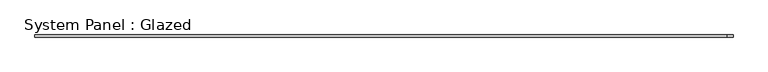
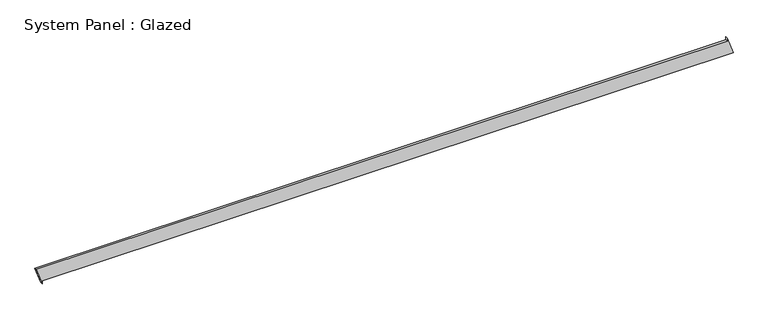
"""IFC4 building model written with IfcOpenShell, lengths in millimetres: plate geometry, System Panel : Glazed."""

import ifcopenshell
import ifcopenshell.guid

model = None  # the IFC model being written
_history = None  # IfcOwnerHistory: only IFC2X3 demands one
_inside = {}  # id of a spatial element -> (the spatial element, [elements in it])
_under = {}  # id of a project, library or spatial element -> (it, [spatial elements below it])
_declared = {}  # id of a project -> (the project, [libraries it declares])
_typed = {}  # id of a type object -> (the type object, [elements of that type])
_made_of = {}  # id of a material, layer set ... -> (it, [elements and type objects made of it])


def new_model(schema):
    """Start an empty IFC model of exactly this schema.

    Asked for "IFC4X3", IfcOpenShell would pick the latest addendum, in which some entities
    have other attributes; the version numbers below select the first issue.
    IFC2X3 requires an IfcOwnerHistory on every rooted entity: one is made here for all.
    """
    global model, _history
    if schema == "IFC4X3":
        model = ifcopenshell.file(schema_version=(4, 3, 0, 0))
    else:
        model = ifcopenshell.file(schema=schema)
    _inside.clear()
    _under.clear()
    _declared.clear()
    _typed.clear()
    _made_of.clear()
    _history = None
    if model.schema == "IFC2X3":
        org = make("IfcOrganization", Name="unknown")
        user = make(
            "IfcPersonAndOrganization",
            ThePerson=make("IfcPerson", FamilyName="unknown"),
            TheOrganization=org,
        )
        app = make(
            "IfcApplication",
            ApplicationDeveloper=org,
            Version="unknown",
            ApplicationFullName="unknown",
            ApplicationIdentifier="unknown",
        )
        _history = make(
            "IfcOwnerHistory",
            OwningUser=user,
            OwningApplication=app,
            ChangeAction="ADDED",
            CreationDate=0,
        )
    return model


def make(cls, **values):
    """One entity of the class cls with the attributes given. An attribute that is None is left unset."""
    return model.create_entity(
        cls, **{name: value for name, value in values.items() if value is not None}
    )


def rooted(cls, **values):
    """An entity with a GlobalId (a new one), such as an element, a storey or a relation."""
    return make(cls, GlobalId=ifcopenshell.guid.new(), OwnerHistory=_history, **values)


def si_unit(unit_type, name, prefix=None):
    """IfcSIUnit, for example si_unit("LENGTHUNIT", "METRE", prefix="MILLI")."""
    return make("IfcSIUnit", UnitType=unit_type, Prefix=prefix, Name=name)


def assignment(units):
    """IfcUnitAssignment: the units of a project."""
    return None if units is None else make("IfcUnitAssignment", Units=units)


def point(xyz):
    """IfcCartesianPoint."""
    return None if xyz is None else make("IfcCartesianPoint", Coordinates=xyz)


def direction(xyz):
    """IfcDirection."""
    return None if xyz is None else make("IfcDirection", DirectionRatios=xyz)


def frame(location, z_axis=None, x_axis=None):
    """IfcAxis2Placement3D, a coordinate frame: its origin and axes. An axis left out is left unset."""
    return make(
        "IfcAxis2Placement3D",
        Location=point(location),
        Axis=direction(z_axis),
        RefDirection=direction(x_axis),
    )


def origin():
    """The frame at (0, 0, 0) with its axes left unset."""
    return frame((0.0, 0.0, 0.0))


def place(relative_to, where):
    """IfcLocalPlacement: puts the frame where relative to a parent placement (None: the world)."""
    return make(
        "IfcLocalPlacement", PlacementRelTo=relative_to, RelativePlacement=where
    )


def context(
    kind, dimensions, precision=None, world=None, true_north=None, identifier=None
):
    """IfcGeometricRepresentationContext, for example the 3D "Model" context."""
    return make(
        "IfcGeometricRepresentationContext",
        ContextIdentifier=identifier,
        ContextType=kind,
        CoordinateSpaceDimension=dimensions,
        Precision=precision,
        WorldCoordinateSystem=world,
        TrueNorth=true_north,
    )


def project(units=None, contexts=None):
    """IfcProject with its units and contexts."""
    return rooted(
        "IfcProject",
        Name="project",
        RepresentationContexts=contexts,
        UnitsInContext=assignment(units),
    )


def spatial(cls, under=None, at=None, **own):
    """A site, building, storey or space (cls), placed at a placement, below another one or the project."""
    s = rooted(cls, ObjectPlacement=at, **own)
    if under is not None:
        _under.setdefault(under.id(), (under, []))[1].append(s)
    return s


def polyline(points):
    """IfcPolyline through the points."""
    return make("IfcPolyline", Points=[point(p) for p in points])


def outline(outer, holes=None, kind="AREA"):
    """IfcArbitraryClosedProfileDef: a profile drawn as a closed curve; with holes, ...WithVoids."""
    if holes is None:
        return make("IfcArbitraryClosedProfileDef", ProfileType=kind, OuterCurve=outer)
    return make(
        "IfcArbitraryProfileDefWithVoids",
        ProfileType=kind,
        OuterCurve=outer,
        InnerCurves=holes,
    )


def extrude(swept, where, along, depth):
    """IfcExtrudedAreaSolid: the profile swept, set in the frame where, extruded along a direction by depth."""
    return make(
        "IfcExtrudedAreaSolid",
        SweptArea=swept,
        Position=where,
        ExtrudedDirection=direction(along),
        Depth=depth,
    )


def shape(context_of_items, identifier, shape_type, items):
    """IfcShapeRepresentation: the items that make up one representation, for example the "Body"."""
    return make(
        "IfcShapeRepresentation",
        ContextOfItems=context_of_items,
        RepresentationIdentifier=identifier,
        RepresentationType=shape_type,
        Items=items,
    )


def source(mapping_origin, context_of_items, identifier, shape_type, items):
    """IfcRepresentationMap: a shape defined once, which mapped items show again and again."""
    return make(
        "IfcRepresentationMap",
        MappingOrigin=mapping_origin,
        MappedRepresentation=shape(context_of_items, identifier, shape_type, items),
    )


def transform(
    local_origin,
    x_axis=None,
    y_axis=None,
    z_axis=None,
    scale=None,
    scale2=None,
    scale3=None,
    uniform=True,
):
    """IfcCartesianTransformationOperator3D, or its non-uniform kind. x_axis, y_axis, z_axis: its Axis1, 2, 3."""
    if uniform:
        return make(
            "IfcCartesianTransformationOperator3D",
            Axis1=direction(x_axis),
            Axis2=direction(y_axis),
            LocalOrigin=point(local_origin),
            Scale=scale,
            Axis3=direction(z_axis),
        )
    return make(
        "IfcCartesianTransformationOperator3DnonUniform",
        Axis1=direction(x_axis),
        Axis2=direction(y_axis),
        LocalOrigin=point(local_origin),
        Scale=scale,
        Axis3=direction(z_axis),
        Scale2=scale2,
        Scale3=scale3,
    )


def mapped(mapping_source, mapping_target):
    """IfcMappedItem: shows the shape of a source again, moved by a transform."""
    return make(
        "IfcMappedItem", MappingSource=mapping_source, MappingTarget=mapping_target
    )


def made_of(thing, what):
    """Note that an element or type object is made of a material, layer set ...; save() writes the relation."""
    if what is not None:
        _made_of.setdefault(what.id(), (what, []))[1].append(thing)
    return thing


def element(
    cls,
    number,
    at=None,
    inside=None,
    cuts=None,
    type_object=None,
    material=None,
    context=None,
    identifier="Body",
    shape_type=None,
    held_by="IfcProductDefinitionShape",
    body=None,
    shapes=None,
    **own,
):
    """One element of the class cls, such as IfcWall. Its Tag is "e" and its number.

    at: its placement. inside: the storey or other place that contains it. cuts: it is an
    opening in that element (IfcRelVoidsElement). A single representation is given by context,
    identifier, shape_type and body (its items); several are given by shapes. held_by: the class
    of the entity that holds the representations. save() writes the other relations.
    """
    e = rooted(cls, Tag="e%d" % number, ObjectPlacement=at, **own)
    if body is not None:
        shapes = [shape(context, identifier, shape_type, body)]
    if shapes is not None:
        e.Representation = make(held_by, Representations=shapes)
    if inside is not None:
        _inside.setdefault(inside.id(), (inside, []))[1].append(e)
    if cuts is not None:
        rooted(
            "IfcRelVoidsElement", RelatingBuildingElement=cuts, RelatedOpeningElement=e
        )
    if type_object is not None:
        _typed.setdefault(type_object.id(), (type_object, []))[1].append(e)
    return made_of(e, material)


def aggregate(whole, parts):
    """IfcRelAggregates: a whole, such as a stair, and the parts it consists of."""
    return rooted("IfcRelAggregates", RelatingObject=whole, RelatedObjects=parts)


def save(model, path):
    """Write the relations noted so far, then the file.

    IfcRelAggregates (storeys below a building ...), IfcRelContainedInSpatialStructure (elements
    in a storey), IfcRelDefinesByType, IfcRelAssociatesMaterial and IfcRelDeclares: one each for
    every whole, place, type object, material and project.
    """
    for whole, parts in _under.values():
        aggregate(whole, parts)
    for where, things in _inside.values():
        rooted(
            "IfcRelContainedInSpatialStructure",
            RelatedElements=things,
            RelatingStructure=where,
        )
    for kind, things in _typed.values():
        rooted("IfcRelDefinesByType", RelatedObjects=things, RelatingType=kind)
    for what, things in _made_of.values():
        rooted("IfcRelAssociatesMaterial", RelatedObjects=things, RelatingMaterial=what)
    for by, libraries in _declared.values():
        rooted("IfcRelDeclares", RelatingContext=by, RelatedDefinitions=libraries)
    model.write(path)


def system_panel_glazed_1d5d9c82(model_context):
    return source(origin(), model_context, "Body", "SweptSolid", [
        extrude(outline(polyline([(0.0, -3957.7762608), (35.3553391, -3957.7762608), (35.3553391, 4027.3165452), (235.5515472, 3958.146555), (200.1962081, 3958.1472368), (200.0422004, -4027.3165452), (0.0, -3957.7762608)])), frame((0.0, -49.5, 0.0), z_axis=(0.0, 1.0, 0.0), x_axis=(0.0, 0.0, 1.0)), (0.0, 0.0, 1.0), 25.0),
    ])


if __name__ == "__main__":
    model = new_model("IFC4")
    model_context = context("Model", 3, world=origin())
    ifc_project = project(units=[si_unit("LENGTHUNIT", "METRE", prefix="MILLI")], contexts=[model_context])
    site = spatial("IfcSite", under=ifc_project)
    building = spatial("IfcBuilding", under=site)
    placement = place(None, origin())
    system_panel_glazed_shape = system_panel_glazed_1d5d9c82(model_context)
    element("IfcPlate", 1, ObjectType="System Panel : Glazed", at=placement, inside=building, context=model_context, shape_type="MappedRepresentation", body=[
        mapped(system_panel_glazed_shape, transform((0.0, 0.0, 0.0), x_axis=(1.0, 0.0, 0.0), y_axis=(0.0, 1.0, 0.0), z_axis=(0.0, 0.0, 1.0))),
    ])
    save(model, "model.ifc")

# Revit data of these elements
# Element 1 (IfcPlate, "System Panel : Glazed")
#   Materials on its faces: "Glass"
# Materials
#   "Glass": class "Glass", colour RGB 218 227 224, transparency 0.85, Description = "Soda Lime Glass", Cost = 0
